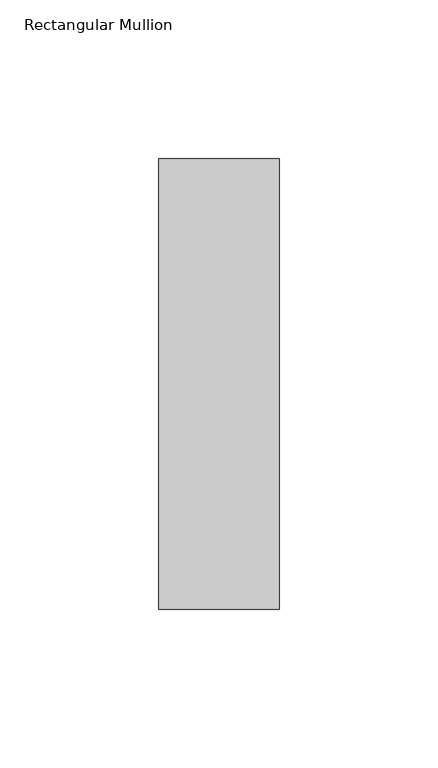
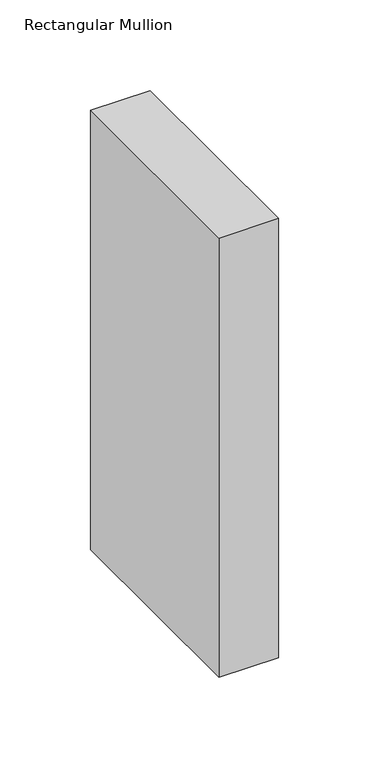
"""IFC4 building model written with IfcOpenShell, lengths in millimetres: member geometry, Rectangular Mullion : NLRS_21_CWM_hsb-regel 38x142_gen_rsf."""

from ifc_helpers import new_model, si_unit, frame, origin, place, context, project, spatial, polyline, outline, extrude, source, transform, mapped, element, save


def rectangular_mullion_67144ce8(model_context):
    return source(origin(), model_context, "Body", "SweptSolid", [
        extrude(outline(polyline([(19.0, -71.0), (-19.0, -71.0), (-19.0, 71.0), (19.0, 71.0), (19.0, -71.0)])), frame((0.0, 0.0, -296.0), z_axis=(0.0, 0.0, 1.0), x_axis=(1.0, 0.0, 0.0)), (0.0, 0.0, 1.0), 296.0),
    ])


if __name__ == "__main__":
    model = new_model("IFC4")
    model_context = context("Model", 3, world=origin())
    ifc_project = project(units=[si_unit("LENGTHUNIT", "METRE", prefix="MILLI")], contexts=[model_context])
    site = spatial("IfcSite", under=ifc_project)
    building = spatial("IfcBuilding", under=site)
    placement = place(None, origin())
    rectangular_mullion_shape = rectangular_mullion_67144ce8(model_context)
    element("IfcMember", 1, ObjectType="Rectangular Mullion : NLRS_21_CWM_hsb-regel 38x142_gen_rsf", at=placement, inside=building, context=model_context, shape_type="MappedRepresentation", body=[
        mapped(rectangular_mullion_shape, transform((0.0, 0.0, 0.0), x_axis=(1.0, 0.0, 0.0), y_axis=(0.0, 1.0, 0.0), z_axis=(0.0, 0.0, 1.0))),
    ])
    save(model, "model.ifc")

# Revit data of these elements
# Type "Rectangular Mullion : NLRS_21_CWM_hsb-regel 38x142_gen_rsf"
#   Export Type to IFC As = "IfcWall"
#   Type IfcGUID = "07M7mRoiH1CR8m_RSKIwpF"
#   Assembly Code = "21.10"
#   built-in parameter 1007322 = 0.465879 (stored number, unit not read)
#   built-in parameter 1007321 = 0.062336 (stored number, unit not read)
#   built-in parameter 1007320 = 0.062336 (stored number, unit not read)
# Element 1 (IfcMember, "Rectangular Mullion : NLRS_21_CWM_hsb-regel 38x142_gen_rsf")
#   Materials on its faces: "NLRS_i2_hout naaldhout vuren_gen_rsf"
# Materials
#   "NLRS_i2_hout naaldhout vuren_gen_rsf": class "I - Hout", colour RGB 234 199 147, transparency 0, Keynote = "i2", Manufacturer = "Revit Standards Foundation", URL = "www.revitstandards.org", Description = "hout vuren", Cost = 0
